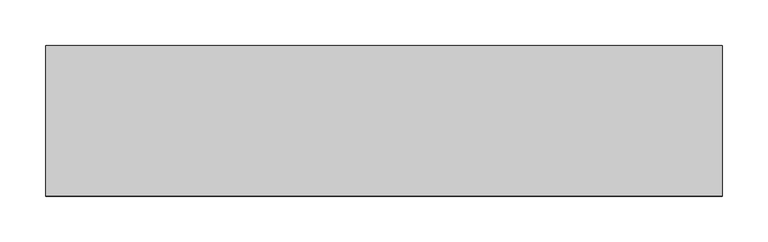
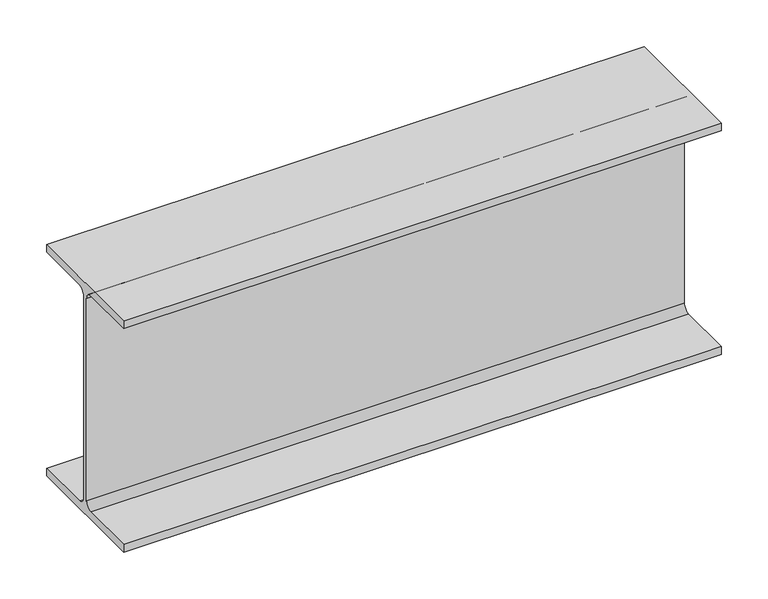
"""IFC4 building model written with IfcOpenShell, lengths in millimetres: beam geometry, Old_Steel Beam_H-KSD3502 : H_SB_ASB_H-300×300x10x15."""

from ifc_helpers import new_model, si_unit, point, frame, frame_2d, origin, place, context, project, spatial, polyline, circle_curve, trimmed, segment, composite_curve, outline, extrude, source, transform, mapped, element, save


def beam_7eb60fd0(model_context):
    return source(origin(), model_context, "Body", "SweptSolid", [
        extrude(outline(composite_curve([segment(polyline([(82.5, -141.5), (82.5, -151.7), (-82.5, -151.7), (-82.5, -141.5), (-11.9, -141.5)]), True, "CONTINUOUS"), segment(trimmed(circle_curve(frame_2d((-11.9, -132.6)), 8.9), [point((-11.9, -141.5))], [point((-3.0, -132.6))], True, "CARTESIAN"), True, "CONTINUOUS"), segment(polyline([(-3.0, -132.6), (-3.0, 132.6)]), True, "CONTINUOUS"), segment(trimmed(circle_curve(frame_2d((-11.9, 132.6)), 8.9), [point((-3.0, 132.6))], [point((-11.9, 141.5))], True, "CARTESIAN"), True, "CONTINUOUS"), segment(polyline([(-11.9, 141.5), (-82.5, 141.5), (-82.5, 151.7), (82.5, 151.7), (82.5, 141.5), (11.9, 141.5)]), True, "CONTINUOUS"), segment(trimmed(circle_curve(frame_2d((11.9, 132.6)), 8.9), [point((11.9, 141.5))], [point((3.0, 132.6))], True, "CARTESIAN"), True, "CONTINUOUS"), segment(polyline([(3.0, 132.6), (3.0, -132.6)]), True, "CONTINUOUS"), segment(trimmed(circle_curve(frame_2d((11.9, -132.6)), 8.9), [point((3.0, -132.6))], [point((11.9, -141.5))], True, "CARTESIAN"), True, "CONTINUOUS"), segment(polyline([(11.9, -141.5), (82.5, -141.5)]), True, "CONTINUOUS")], self_intersect=False)), frame((-237.9749298, 0.0, 0.0), z_axis=(1.0, 0.0, 0.0), x_axis=(0.0, 1.0, 0.0)), (0.0, 0.0, 1.0), 740.4687108),
    ])


if __name__ == "__main__":
    model = new_model("IFC4")
    model_context = context("Model", 3, world=origin())
    ifc_project = project(units=[si_unit("LENGTHUNIT", "METRE", prefix="MILLI")], contexts=[model_context])
    site = spatial("IfcSite", under=ifc_project)
    building = spatial("IfcBuilding", under=site)
    placement = place(None, origin())
    beam_shape = beam_7eb60fd0(model_context)
    element("IfcBeam", 1, ObjectType="Old_Steel Beam_H-KSD3502 : H_SB_ASB_H-300×300x10x15", at=placement, inside=building, context=model_context, shape_type="MappedRepresentation", body=[
        mapped(beam_shape, transform((0.0, 0.0, 0.0), x_axis=(1.0, 0.0, 0.0), y_axis=(0.0, 1.0, 0.0), z_axis=(0.0, 0.0, 1.0))),
    ])
    save(model, "model.ifc")

# Revit data of these elements
# Type "Old_Steel Beam_H-KSD3502 : H_SB_ASB_H-300×300x10x15"
#   Width = 30.0 cm
#   Web Thickness = 1.0 cm
#   Web Fillet = 1.8 cm
#   Warping Constant = 1370670.0 cm⁶
#   Torsional Moment of Inertia = 77.00 cm⁴
#   Torsional Modulus = 1.0 cm³
#   Section Area = 119.8 cm²
#   Plastic Modulus weak axis = 684.0 cm³
#   Plastic Modulus strong axis = 1500.0 cm³
#   Perimeter = 1.75 m²/m
#   Nominal Weight = 94.00 kgf/m
#   Moment of Inertia weak axis = 6750.00 cm⁴
#   Moment of Inertia strong axis = 20400.00 cm⁴
#   Height = 30.0 cm
#   Flange Thickness = 1.5 cm
#   Elastic Modulus weak axis = 450.0 cm³
#   Elastic Modulus strong axis = 1360.0 cm³
#   Centroid Vertical = 15.0 cm
#   Centroid Horizontal = 15.0 cm
#   Length [instance default] = 1.5240 m
#   Structural Material [instance default] = Steel, 45-345
#   Assembly Code = ""
# Element 1 (IfcBeam, "Old_Steel Beam_H-KSD3502 : H_SB_ASB_H-300×300x10x15")
#   Structural Material = none
# Materials
#   "Steel, 45-345": class "Metal", colour RGB 189 187 185, transparency 0, Description = "Steel 345 MPa", Cost = 0
